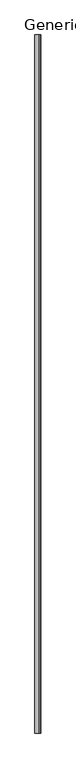
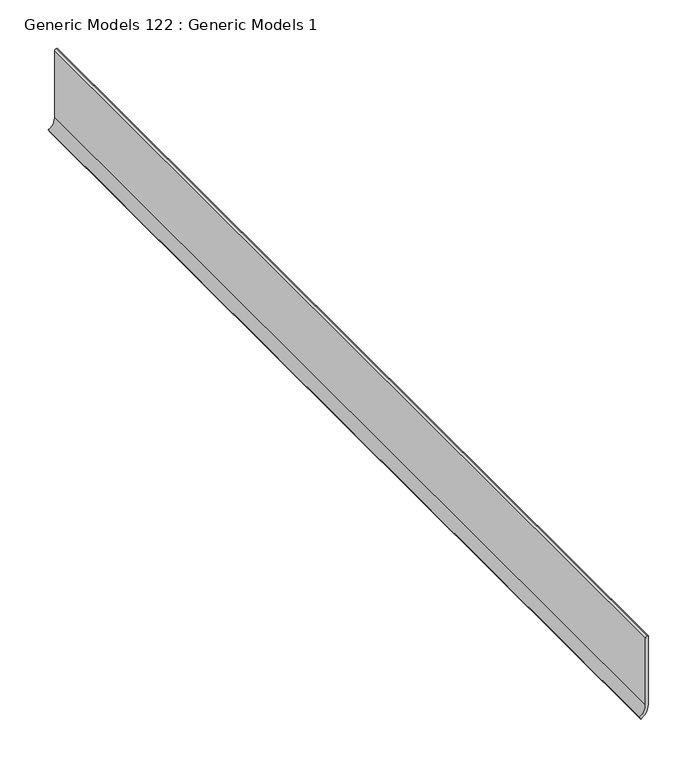
"""IFC4 building model written with IfcOpenShell, lengths in millimetres: proxy geometry, Generic Models 122 : Generic Models 1."""

from ifc_helpers import new_model, si_unit, point, frame, frame_2d, origin, place, context, project, spatial, polyline, circle_curve, trimmed, segment, composite_curve, outline, extrude, source, transform, mapped, element, save


def generic_models_122_generic_models_1_fdd6cadd(model_context):
    return source(origin(), model_context, "Body", "SweptSolid", [
        extrude(outline(composite_curve([segment(polyline([(73.749588, 48367.3939813), (73.749588, 48366.3057831)]), True, "CONTINUOUS"), segment(trimmed(circle_curve(frame_2d((71.6627862, 48366.3057831)), 2.0868018), [point((73.749588, 48366.3057831))], [point((71.6627862, 48364.2189813))], False, "CARTESIAN"), True, "CONTINUOUS"), segment(polyline([(71.6627862, 48364.2189813), (-12.4007813, 48364.2189813)]), True, "CONTINUOUS"), segment(trimmed(circle_curve(frame_2d((-12.4007813, 48349.5542845)), 14.6646968), [point((-12.4007813, 48364.2189813))], [point((-25.1007813, 48356.8866329))], True, "CARTESIAN"), True, "CONTINUOUS"), segment(polyline([(-25.1007813, 48356.8866329), (-27.850412, 48358.4741329)]), True, "CONTINUOUS"), segment(trimmed(circle_curve(frame_2d((-12.4007813, 48349.5542845)), 17.8396968), [point((-27.850412, 48358.4741329))], [point((-12.4007813, 48367.3939813))], False, "CARTESIAN"), True, "CONTINUOUS"), segment(polyline([(-12.4007813, 48367.3939813), (73.749588, 48367.3939813)]), True, "CONTINUOUS")], self_intersect=False)), frame((0.0, 0.0, 0.0), z_axis=(0.0, 1.0, 0.0), x_axis=(0.0, 0.0, 1.0)), (0.0, 0.0, 1.0), 1219.2),
    ])


if __name__ == "__main__":
    model = new_model("IFC4")
    model_context = context("Model", 3, world=origin())
    ifc_project = project(units=[si_unit("LENGTHUNIT", "METRE", prefix="MILLI")], contexts=[model_context])
    site = spatial("IfcSite", under=ifc_project)
    building = spatial("IfcBuilding", under=site)
    placement = place(None, origin())
    generic_models_122_generic_models_1_shape = generic_models_122_generic_models_1_fdd6cadd(model_context)
    element("IfcBuildingElementProxy", 1, Name="Generic Models 122 : Generic Models 1", ObjectType="Generic Models 122 : Generic Models 1", at=placement, inside=building, context=model_context, shape_type="MappedRepresentation", body=[
        mapped(generic_models_122_generic_models_1_shape, transform((0.0, 0.0, 0.0), x_axis=(1.0, 0.0, 0.0), y_axis=(0.0, 1.0, 0.0), z_axis=(0.0, 0.0, 1.0))),
    ])
    save(model, "model.ifc")

# Revit data of these elements
# Element 1 (IfcBuildingElementProxy, "Generic Models 122 : Generic Models 1")
#   Materials on its faces: "BASE AS SCHEDULED"
# Materials
#   "BASE AS SCHEDULED": class "Generic", colour RGB 120 120 120, transparency 0, Cost = 0
